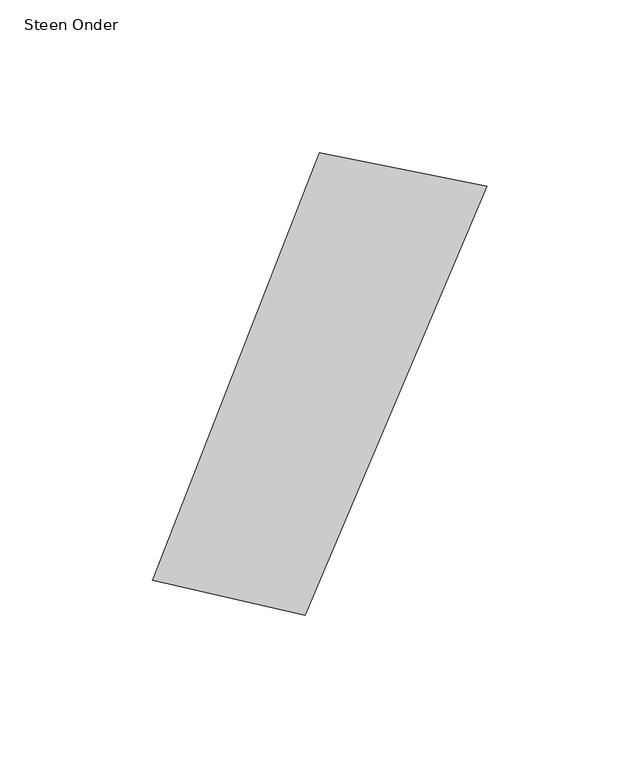
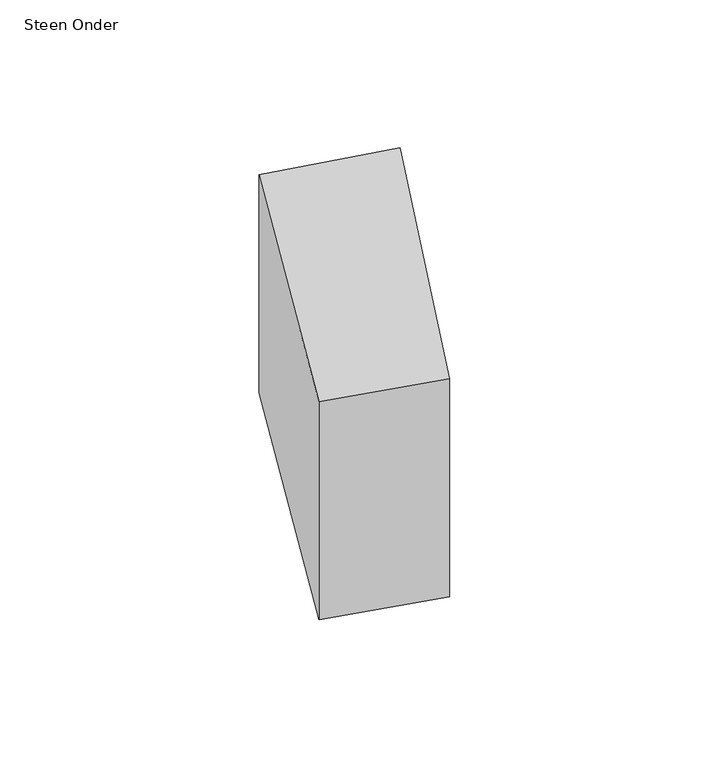
"""IFC4 building model written with IfcOpenShell, lengths in millimetres: proxy geometry, 00_GMA_steen_versie_4 : Steen Onder."""

from ifc_helpers import new_model, si_unit, origin, origin_with_axes, place, context, project, spatial, polyline, outline, extrude, source, transform, mapped, element, save


def steen_onder_7f6a3932(model_context):
    return source(origin(), model_context, "Body", "SweptSolid", [
        extrude(outline(polyline([(129.5386538, 137.6891273), (69.8620933, -2.9000965), (19.8811924, 8.6301255), (74.55433, 148.6462189), (129.5386538, 137.6891273)])), origin_with_axes(), (0.0, 0.0, 1.0), 100.0),
    ])


if __name__ == "__main__":
    model = new_model("IFC4")
    model_context = context("Model", 3, world=origin())
    ifc_project = project(units=[si_unit("LENGTHUNIT", "METRE", prefix="MILLI")], contexts=[model_context])
    site = spatial("IfcSite", under=ifc_project)
    building = spatial("IfcBuilding", under=site)
    placement = place(None, origin())
    steen_onder_shape = steen_onder_7f6a3932(model_context)
    element("IfcBuildingElementProxy", 1, Name="00_GMA_steen_versie_4 : Steen Onder", ObjectType="00_GMA_steen_versie_4 : Steen Onder", at=placement, inside=building, context=model_context, shape_type="MappedRepresentation", body=[
        mapped(steen_onder_shape, transform((0.0, 0.0, 0.0), x_axis=(1.0, 0.0, 0.0), y_axis=(0.0, 1.0, 0.0), z_axis=(0.0, 0.0, 1.0))),
    ])
    save(model, "model.ifc")

# Revit data of these elements
# Type "00_GMA_steen_versie_4 : Steen Onder"
#   StootVoegHalfBoven [instance default] = 5 mm
#   StootVoegHalf [instance default] = 5 mm
#   StootVoegBreedteOnder = 10 mm
#   StootVoegBreedteBoven = 10 mm
#   Steendikte = 100 mm
#   LintVoegOnderHalf = 0 mm
#   LintVoegOnder = 0 mm
#   LintVoegBovenHalf = 5 mm
#   LintVoegBoven = 10 mm
#   materiaal = none
#   MateriaalVoeg = none
#   Default Elevation = 0
